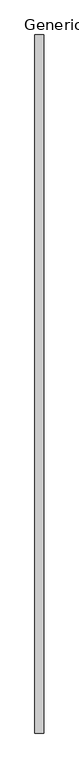
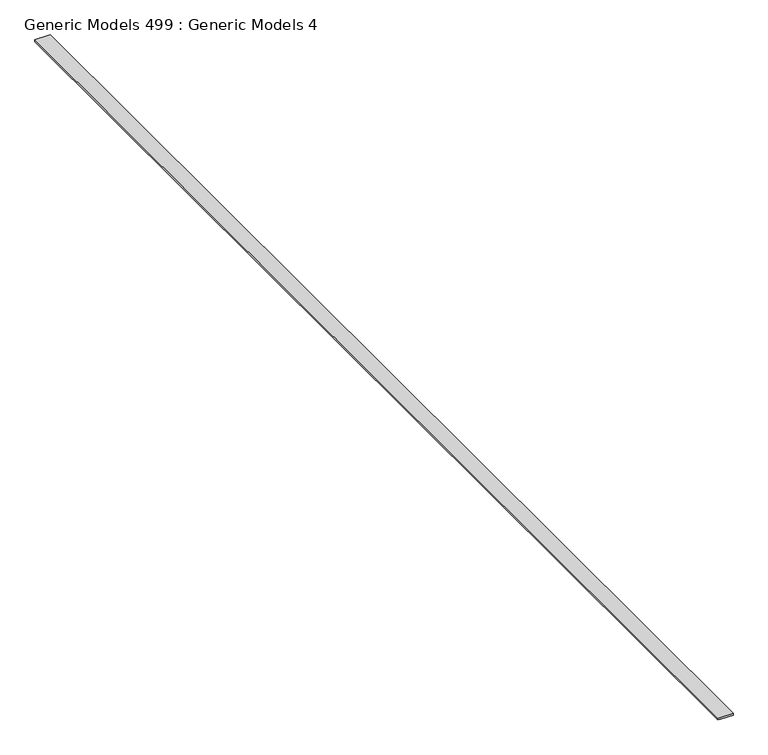
"""IFC4 building model written with IfcOpenShell, lengths in millimetres: proxy geometry, Generic Models 499 : Generic Models 4."""

from ifc_helpers import new_model, si_unit, origin, place, context, project, spatial, faceted_brep, source, transform, mapped, element, save


def generic_models_499_generic_models_4_27303224(model_context):
    return source(origin(), model_context, "Body", "Brep", [
        faceted_brep([(-8006.0475369, -464.1230338, 126364.746), (-8162.2575369, -464.1230338, 126364.746), (-8162.2575369, -464.1230338, 126355.221), (-8162.2575369, -464.1230338, 126343.791), (-8139.814353, -464.1230338, 126343.791), (-8139.814353, -464.1230338, 126342.521), (-8006.0475369, -464.1230338, 126342.521), (-8162.2575369, 11778.6769662, 126364.746), (-8006.0475369, 11778.6769662, 126364.746), (-8006.0475369, 11778.6769662, 126342.521), (-8139.814353, 11778.6769662, 126342.521), (-8139.814353, 11778.6769662, 126343.791), (-8162.2575369, 11778.6769662, 126343.791), (-8162.2575369, 11778.6769662, 126355.221)], [[[0, 1, 2, 3, 4, 5, 6]], [[7, 8, 9, 10, 11, 12, 13]], [[1, 0, 8, 7]], [[9, 6, 5, 10]], [[1, 7, 13, 12, 3, 2]], [[0, 6, 9, 8]], [[4, 11, 10, 5]], [[11, 4, 3, 12]]]),
    ])


if __name__ == "__main__":
    model = new_model("IFC4")
    model_context = context("Model", 3, world=origin())
    ifc_project = project(units=[si_unit("LENGTHUNIT", "METRE", prefix="MILLI")], contexts=[model_context])
    site = spatial("IfcSite", under=ifc_project)
    building = spatial("IfcBuilding", under=site)
    placement = place(None, origin())
    generic_models_499_generic_models_4_shape = generic_models_499_generic_models_4_27303224(model_context)
    element("IfcBuildingElementProxy", 1, Name="Generic Models 499 : Generic Models 4", ObjectType="Generic Models 499 : Generic Models 4", at=placement, inside=building, context=model_context, shape_type="MappedRepresentation", body=[
        mapped(generic_models_499_generic_models_4_shape, transform((0.0, 0.0, 0.0), x_axis=(1.0, 0.0, 0.0), y_axis=(0.0, 1.0, 0.0), z_axis=(0.0, 0.0, 1.0))),
    ])
    save(model, "model.ifc")

# Revit data of these elements
# Element 1 (IfcBuildingElementProxy, "Generic Models 499 : Generic Models 4")
#   Materials on its faces: "_7/8\" SMOOTH TROWEL EXTERIOR STUCCO (COLOR PER OWNER)"
# Materials
#   "_7/8\" SMOOTH TROWEL EXTERIOR STUCCO (COLOR PER OWNER)": class "Generic", colour RGB 233 233 233, transparency 0, Cost = 0
